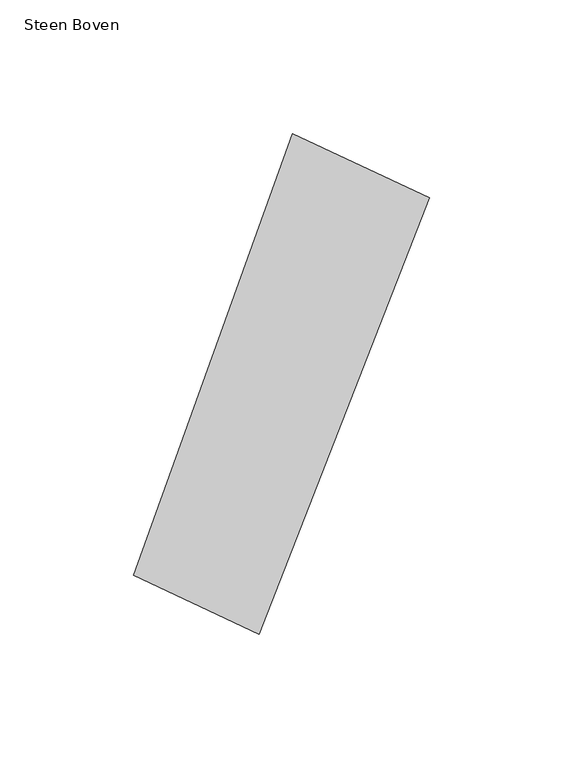
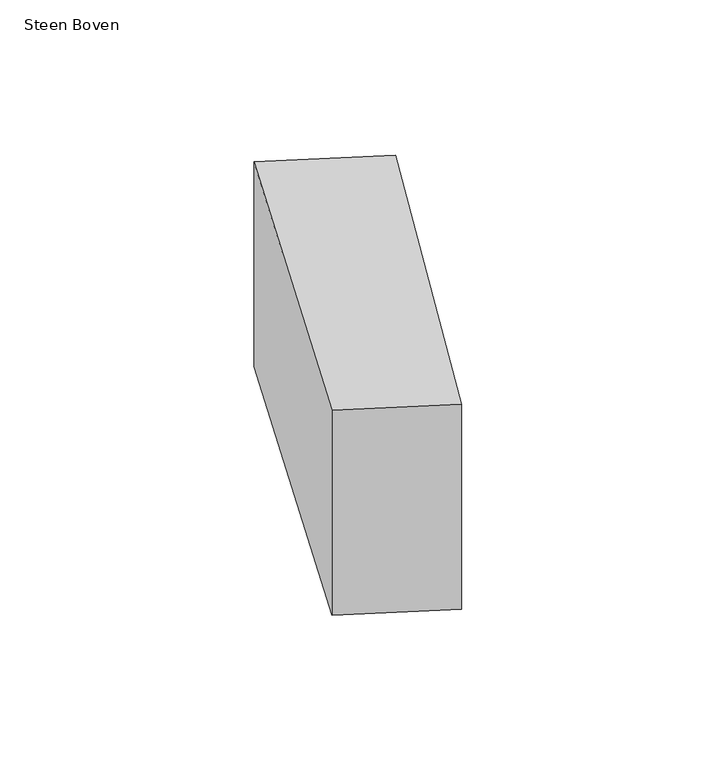
"""IFC4 building model written with IfcOpenShell, lengths in millimetres: proxy geometry, 00_GMA_steen_versie_4 : Steen Boven."""

from ifc_helpers import new_model, si_unit, origin, origin_with_axes, place, context, project, spatial, polyline, outline, extrude, source, transform, mapped, element, save


def steen_boven_51b12e60(model_context):
    return source(origin(), model_context, "Body", "SweptSolid", [
        extrude(outline(polyline([(133.8474479, 154.7382254), (70.0258973, -8.6389831), (22.9536082, 13.4532429), (82.5535619, 178.8224188), (133.8474479, 154.7382254)])), origin_with_axes(), (0.0, 0.0, 1.0), 100.0),
    ])


if __name__ == "__main__":
    model = new_model("IFC4")
    model_context = context("Model", 3, world=origin())
    ifc_project = project(units=[si_unit("LENGTHUNIT", "METRE", prefix="MILLI")], contexts=[model_context])
    site = spatial("IfcSite", under=ifc_project)
    building = spatial("IfcBuilding", under=site)
    placement = place(None, origin())
    steen_boven_shape = steen_boven_51b12e60(model_context)
    element("IfcBuildingElementProxy", 1, Name="00_GMA_steen_versie_4 : Steen Boven", ObjectType="00_GMA_steen_versie_4 : Steen Boven", at=placement, inside=building, context=model_context, shape_type="MappedRepresentation", body=[
        mapped(steen_boven_shape, transform((0.0, 0.0, 0.0), x_axis=(1.0, 0.0, 0.0), y_axis=(0.0, 1.0, 0.0), z_axis=(0.0, 0.0, 1.0))),
    ])
    save(model, "model.ifc")

# Revit data of these elements
# Type "00_GMA_steen_versie_4 : Steen Boven"
#   StootVoegHalfBoven [instance default] = 5 mm
#   StootVoegHalf [instance default] = 5 mm
#   StootVoegBreedteOnder = 10 mm
#   StootVoegBreedteBoven = 10 mm
#   Steendikte = 100 mm
#   LintVoegOnderHalf = 5 mm
#   LintVoegOnder = 10 mm
#   LintVoegBovenHalf = 0 mm
#   LintVoegBoven = 0 mm
#   materiaal = none
#   MateriaalVoeg = none
#   Default Elevation = 0
